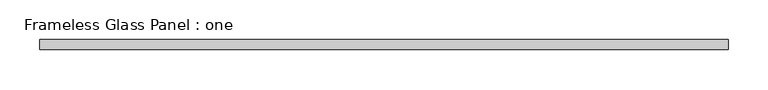
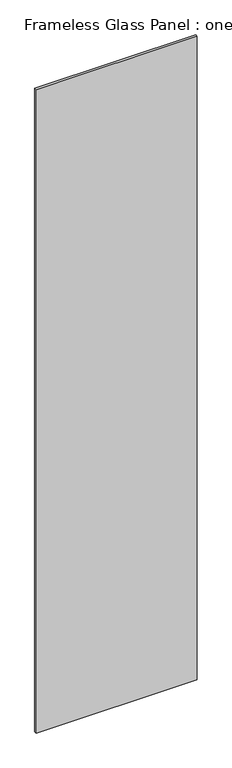
"""IFC4 building model written with IfcOpenShell, lengths in millimetres: plate geometry, Frameless Glass Panel : one."""

from ifc_helpers import new_model, si_unit, origin, origin_with_axes, place, context, project, spatial, polyline, outline, extrude, source, transform, mapped, element, save


def frameless_glass_panel_one_7a78a32b(model_context):
    return source(origin(), model_context, "Body", "SweptSolid", [
        extrude(outline(polyline([(432.5666196, -6.35), (-432.5666196, -6.35), (-432.5666196, 6.35), (432.5666196, 6.35), (432.5666196, -6.35)])), origin_with_axes(), (0.0, 0.0, 1.0), 3651.25),
    ])


if __name__ == "__main__":
    model = new_model("IFC4")
    model_context = context("Model", 3, world=origin())
    ifc_project = project(units=[si_unit("LENGTHUNIT", "METRE", prefix="MILLI")], contexts=[model_context])
    site = spatial("IfcSite", under=ifc_project)
    building = spatial("IfcBuilding", under=site)
    placement = place(None, origin())
    frameless_glass_panel_one_shape = frameless_glass_panel_one_7a78a32b(model_context)
    element("IfcPlate", 1, ObjectType="Frameless Glass Panel : one", at=placement, inside=building, context=model_context, shape_type="MappedRepresentation", body=[
        mapped(frameless_glass_panel_one_shape, transform((0.0, 0.0, 0.0), x_axis=(1.0, 0.0, 0.0), y_axis=(0.0, 1.0, 0.0), z_axis=(0.0, 0.0, 1.0))),
    ])
    save(model, "model.ifc")

# Revit data of these elements
# Type "Frameless Glass Panel : one"
#   Glass Thickness = 0' - 0 1/2"
#   Gap btwn Panels = 0' - 0 1/4"
#   Panel Material = TEMPERED GLASS DOOR/SIDELIGHT TO MATCH EXISTING CONF. ROOM
# Element 1 (IfcPlate, "Frameless Glass Panel : one")
#   Materials on its faces: "TEMPERED GLASS DOOR/SIDELIGHT TO MATCH EXISTING CONF. ROOM"
# Materials
#   "TEMPERED GLASS DOOR/SIDELIGHT TO MATCH EXISTING CONF. ROOM": class "Glass", colour RGB 218 227 224, transparency 0.85, Description = "Soda Lime Glass", Cost = 0
